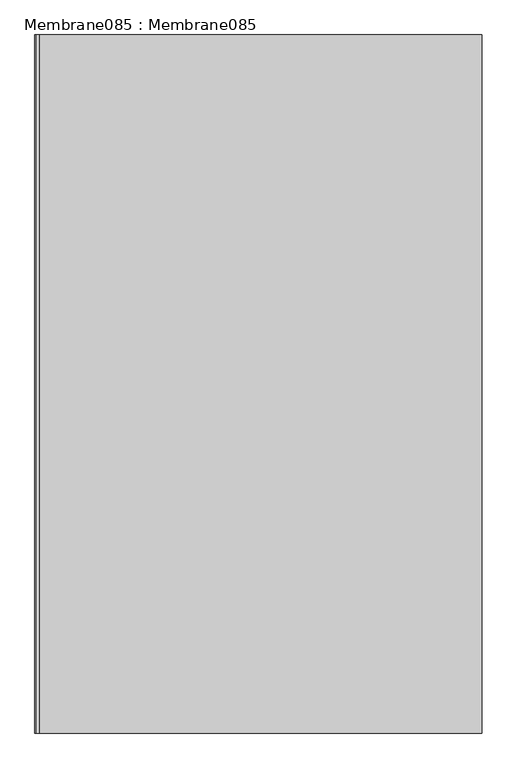
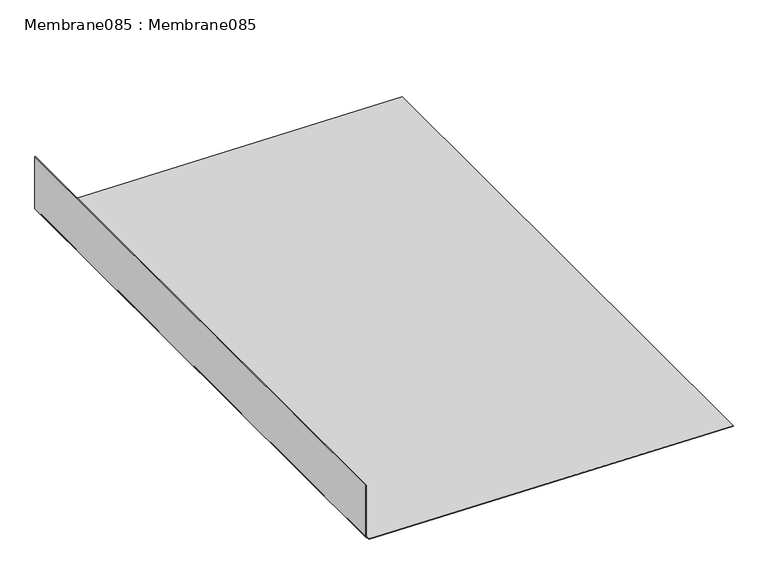
"""IFC4 building model written with IfcOpenShell, lengths in millimetres: proxy geometry, Membrane085 : Membrane085."""

from ifc_helpers import new_model, si_unit, frame, origin, place, context, project, spatial, polyline, outline, extrude, source, transform, mapped, element, save


def membrane085_membrane085_3734e25c(model_context):
    return source(origin(), model_context, "Body", "SweptSolid", [
        extrude(outline(polyline([(40034.453125, 16509.7552564), (40007.906554, 17779.7441406), (40009.8905206, 17779.7856114), (40036.4202235, 16510.603698), (40046.6641063, 16500.5248126), (40238.2890625, 16500.5248126), (40238.2890625, 16498.5404126), (40045.8515625, 16498.5404126), (40034.453125, 16509.7552564)])), frame((0.0, -1052.8906567, 0.0), z_axis=(0.0, 1.0, 0.0), x_axis=(0.0, 0.0, 1.0)), (0.0, 0.0, 1.0), 1999.85),
    ])


if __name__ == "__main__":
    model = new_model("IFC4")
    model_context = context("Model", 3, world=origin())
    ifc_project = project(units=[si_unit("LENGTHUNIT", "METRE", prefix="MILLI")], contexts=[model_context])
    site = spatial("IfcSite", under=ifc_project)
    building = spatial("IfcBuilding", under=site)
    placement = place(None, origin())
    membrane085_membrane085_shape = membrane085_membrane085_3734e25c(model_context)
    element("IfcBuildingElementProxy", 1, Name="Membrane085 : Membrane085", ObjectType="Membrane085 : Membrane085", at=placement, inside=building, context=model_context, shape_type="MappedRepresentation", body=[
        mapped(membrane085_membrane085_shape, transform((0.0, 0.0, 0.0), x_axis=(1.0, 0.0, 0.0), y_axis=(0.0, 1.0, 0.0), z_axis=(0.0, 0.0, 1.0))),
    ])
    save(model, "model.ifc")

# Revit data of these elements
# Type "Membrane085 : Membrane085"
#   NameOverride = "Membrane085"
# Element 1 (IfcBuildingElementProxy, "Membrane085 : Membrane085")
#   Materials on its faces: "WESTCOAT ALX UNDER TILE WATERPROOFING SYSTEM (FOLLOW MANUFACTURER'S INSTALLATION REQUIREMENTS)"
# Materials
#   "WESTCOAT ALX UNDER TILE WATERPROOFING SYSTEM (FOLLOW MANUFACTURER'S INSTALLATION REQUIREMENTS)": class "Unassigned", colour RGB 179 255 168, transparency 0, Cost = 0
